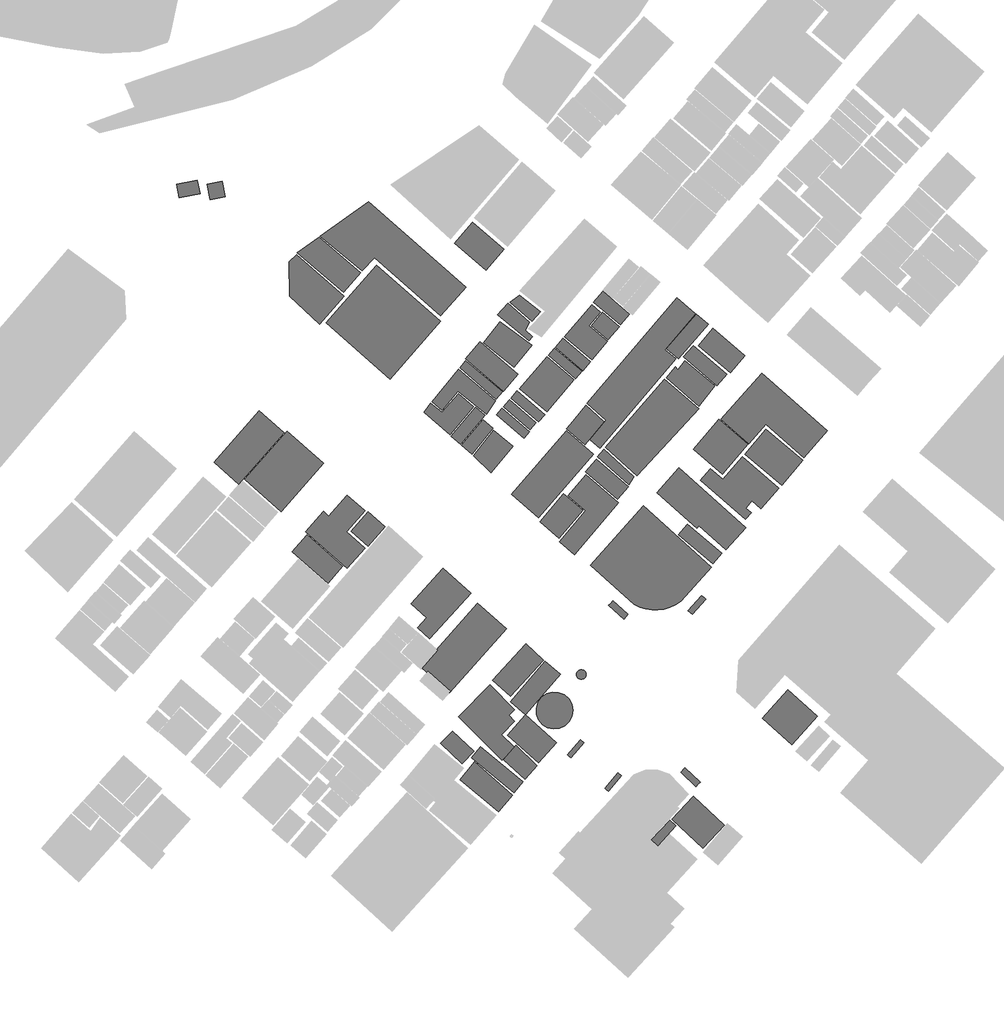
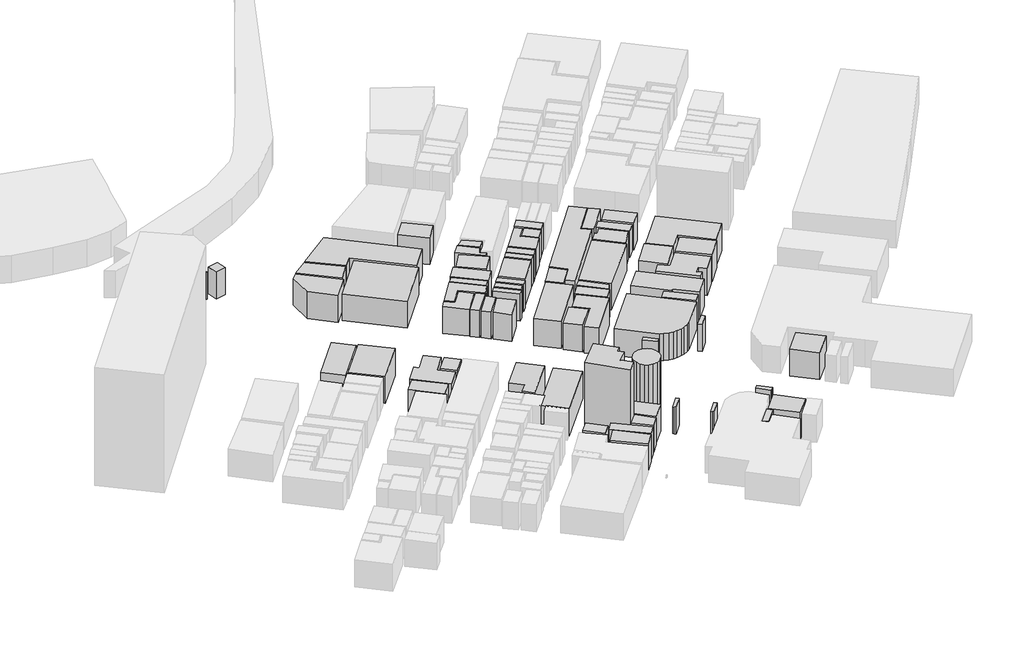
# One storey, part 2 of 3: 70 proxies.
"""IFC4 building model written with IfcOpenShell, lengths in millimetres."""

from ifc_helpers import new_model, si_unit, origin, origin_with_axes, place, context, project, spatial, polyline, outline, extrude, element, save

model = new_model("IFC4")

# Units and contexts
model_context = context("Model", 3, world=origin())
ifc_project = project(units=[si_unit("LENGTHUNIT", "METRE", prefix="MILLI")], contexts=[model_context])

# Site, building, storey
site = spatial("IfcSite", under=ifc_project)
building = spatial("IfcBuilding", under=site)
storey = spatial("IfcBuildingStorey", under=building, Name="レベル 0", Elevation=0.0)

# Proxies
placement = place(None, origin())
element("IfcBuildingElementProxy", 1, Name="Mass", at=placement, inside=storey, context=model_context, shape_type="SweptSolid", body=[
    extrude(outline(polyline([(170698.7323915, 46624.0327425), (171096.1893538, 44511.3291361), (170789.0635192, 42387.5060369), (169804.4542245, 40486.0727911), (168268.8250515, 38984.9412821), (166326.7058014, 38073.1428832), (164194.8911837, 37828.5140449), (162099.2090151, 38284.4132439), (160265.4871197, 39385.2430179), (158883.4208628, 41030.9279318), (158097.5400505, 43054.6755966), (158016.2420351, 45234.096159), (158657.593041, 47313.4412879), (159931.2619458, 49070.3211289), (161719.8182773, 50315.7043068), (163815.500446, 50905.0374178), (165983.4475152, 50782.7229987), (167997.8316659, 49959.8805414), (169623.7919691, 48514.3464955), (170698.7323915, 46624.0327425)])), origin_with_axes(), (0.0, 0.0, 1.0), 35000.0),
])
element("IfcBuildingElementProxy", 2, Name="Mass", at=placement, inside=storey, context=model_context, shape_type="SweptSolid", body=[
    extrude(outline(polyline([(130374.9168956, 42153.9966913), (141485.6456275, 53473.6402233), (150256.798147, 44678.1215256), (148287.5795602, 42676.6128464), (150310.9968231, 40486.0727911), (145677.0099623, 35793.6468872), (150175.5001316, 31245.7743872), (145848.6391053, 26586.7069609), (130374.9168956, 42153.9966913)])), origin_with_axes(), (0.0, 0.0, 1.0), 45000.0),
])
element("IfcBuildingElementProxy", 3, Name="Mass", at=placement, inside=storey, context=model_context, shape_type="SweptSolid", body=[
    extrude(outline(polyline([(208574.5743203, 165836.1135976), (210995.448548, 168927.3325589), (221636.4554144, 160031.7384269), (215927.5281312, 152781.8292102), (204419.3424371, 162933.9260122), (207608.0312501, 166803.5094596), (208574.5743203, 165836.1135976)])), origin_with_axes(), (0.0, 0.0, 1.0), 15000.0),
])
element("IfcBuildingElementProxy", 4, Name="Mass", at=placement, inside=storey, context=model_context, shape_type="SweptSolid", body=[
    extrude(outline(polyline([(177934.2557355, 188964.6583397), (180978.4147472, 186362.6970567), (176868.3484279, 181547.9567328), (183462.5207633, 175921.4934444), (177780.6928194, 169283.1563236), (168151.3945845, 177511.5808958), (177934.2557355, 188964.6583397)])), origin_with_axes(), (0.0, 0.0, 1.0), 15000.0),
])
element("IfcBuildingElementProxy", 5, Name="Mass", at=placement, inside=storey, context=model_context, shape_type="SweptSolid", body=[
    extrude(outline(polyline([(164809.1428529, 173875.5067947), (167519.0766882, 177044.562204), (177310.970954, 168671.5842278), (174601.0371162, 165502.5288177), (164809.1428529, 173875.5067947)])), origin_with_axes(), (0.0, 0.0, 1.0), 15000.0),
])
element("IfcBuildingElementProxy", 6, Name="Mass", at=placement, inside=storey, context=model_context, shape_type="SweptSolid", body=[
    extrude(outline(polyline([(146282.2285192, 152626.1563127), (148432.1093639, 155139.161655), (157980.1095835, 146988.5735315), (155830.2287387, 144475.5681892), (146282.2285192, 152626.1563127)])), origin_with_axes(), (0.0, 0.0, 1.0), 15000.0),
])
element("IfcBuildingElementProxy", 7, Name="Mass", at=placement, inside=storey, context=model_context, shape_type="SweptSolid", body=[
    extrude(outline(polyline([(247760.2176028, 51805.7163239), (258292.8271145, 42287.4306033), (249151.3169721, 32168.6922789), (238618.7074578, 41686.9779995), (247760.2176028, 51805.7163239)])), origin_with_axes(), (0.0, 0.0, 1.0), 15000.0),
])
element("IfcBuildingElementProxy", 8, Name="Mass", at=placement, inside=storey, context=model_context, shape_type="SweptSolid", body=[
    extrude(outline(polyline([(145125.990084, 182937.8933163), (156489.6459718, 174520.4373689), (150148.4007948, 166681.1950405), (139254.4667699, 175421.116275), (145125.990084, 182937.8933163)])), origin_with_axes(), (0.0, 0.0, 1.0), 15000.0),
])
element("IfcBuildingElementProxy", 9, Name="Mass", at=placement, inside=storey, context=model_context, shape_type="SweptSolid", body=[
    extrude(outline(polyline([(139028.6389507, 148000.447364), (142551.5529376, 144864.7504331), (135026.9699836, 135657.8105068), (131350.4930781, 138860.2243936), (139028.6389507, 148000.447364)])), origin_with_axes(), (0.0, 0.0, 1.0), 15000.0),
])
element("IfcBuildingElementProxy", 10, Name="Mass", at=placement, inside=storey, context=model_context, shape_type="SweptSolid", body=[
    extrude(outline(polyline([(215792.0314397, 174387.0034569), (221031.2368575, 180524.9634075), (232394.8927479, 170817.6463118), (227155.6873275, 164679.6863612), (215792.0314397, 174387.0034569)])), origin_with_axes(), (0.0, 0.0, 1.0), 15000.0),
])
element("IfcBuildingElementProxy", 11, Name="Mass", at=placement, inside=storey, context=model_context, shape_type="SweptSolid", body=[
    extrude(outline(polyline([(203868.3225562, 173008.1863662), (207725.4617171, 169716.8165378), (180707.4213617, 137803.8725908), (177220.6398263, 140939.5695225), (182839.2359819, 147878.1329448), (176109.5669524, 153916.0174618), (208177.117358, 191455.4246972), (214798.3890328, 185795.6029305), (203868.3225562, 173008.1863662)])), origin_with_axes(), (0.0, 0.0, 1.0), 15000.0),
])
element("IfcBuildingElementProxy", 12, Name="Mass", at=placement, inside=storey, context=model_context, shape_type="SweptSolid", body=[
    extrude(outline(polyline([(138025.9634289, 175721.3425765), (151422.0696971, 164268.2651325), (146246.0960676, 158219.2611227), (132849.9898021, 169672.3385674), (138025.9634289, 175721.3425765)])), origin_with_axes(), (0.0, 0.0, 1.0), 15000.0),
])
element("IfcBuildingElementProxy", 13, Name="Mass", at=placement, inside=storey, context=model_context, shape_type="SweptSolid", body=[
    extrude(outline(polyline([(162334.0699465, 170951.0802238), (164502.0170183, 173486.3245509), (174230.6794932, 165180.0635306), (172053.6993091, 162633.6997107), (162334.0699465, 170951.0802238)])), origin_with_axes(), (0.0, 0.0, 1.0), 15000.0),
])
element("IfcBuildingElementProxy", 14, Name="Mass", at=placement, inside=storey, context=model_context, shape_type="SweptSolid", body=[
    extrude(outline(polyline([(187355.7923757, 118344.7604281), (171556.8781069, 99930.8805755), (166218.3084467, 104512.1115531), (175630.8119747, 115475.9313204), (169334.732359, 120880.0047552), (175721.1431024, 128318.9453478), (187355.7923757, 118344.7604281)])), origin_with_axes(), (0.0, 0.0, 1.0), 15000.0),
])
element("IfcBuildingElementProxy", 15, Name="Mass", at=placement, inside=storey, context=model_context, shape_type="SweptSolid", body=[
    extrude(outline(polyline([(168792.745593, 144742.4360131), (170156.7456229, 146410.3599133), (175648.8781992, 153137.6529749), (182152.7194095, 147299.9193266), (175323.6861401, 139104.8532327), (168792.745593, 144742.4360131)])), origin_with_axes(), (0.0, 0.0, 1.0), 15000.0),
])
element("IfcBuildingElementProxy", 16, Name="Mass", at=placement, inside=storey, context=model_context, shape_type="SweptSolid", body=[
    extrude(outline(polyline([(144186.5463531, 185328.5842386), (147953.3543863, 189565.1109435), (155676.6658227, 182782.2204187), (154159.1028717, 179813.3158774), (156715.4737935, 177600.5368366), (155333.4075365, 176043.8078635), (144186.5463531, 185328.5842386)])), origin_with_axes(), (0.0, 0.0, 1.0), 15000.0),
])
element("IfcBuildingElementProxy", 17, Name="Mass", at=placement, inside=storey, context=model_context, shape_type="SweptSolid", body=[
    extrude(outline(polyline([(148956.0299055, 155661.77781), (151160.1094263, 158241.5001083), (161060.4010443, 149779.5661905), (158856.3215234, 147199.8438922), (148956.0299055, 155661.77781)])), origin_with_axes(), (0.0, 0.0, 1.0), 15000.0),
])
element("IfcBuildingElementProxy", 18, Name="Mass", at=placement, inside=storey, context=model_context, shape_type="SweptSolid", body=[
    extrude(outline(polyline([(182649.5406117, 138148.5768635), (203660.5609616, 162455.7878276), (216017.8592589, 151903.3892898), (193940.9315989, 128085.4360023), (182649.5406117, 138148.5768635)])), origin_with_axes(), (0.0, 0.0, 1.0), 15000.0),
])
element("IfcBuildingElementProxy", 19, Name="Mass", at=placement, inside=storey, context=model_context, shape_type="SweptSolid", body=[
    extrude(outline(polyline([(143852.3211792, 149790.6856833), (145812.5066538, 152081.3011721), (155622.4671441, 143697.2037031), (153662.2816695, 141395.4687215), (143852.3211792, 149790.6856833)])), origin_with_axes(), (0.0, 0.0, 1.0), 15000.0),
])
element("IfcBuildingElementProxy", 20, Name="Mass", at=placement, inside=storey, context=model_context, shape_type="SweptSolid", body=[
    extrude(outline(polyline([(130230.3870919, 157296.3432318), (135695.4203289, 152537.2003711), (127195.2611949, 142629.7324075), (117945.3536977, 150635.7671254), (120375.2610377, 153838.1810131), (124494.3604693, 150591.289155), (130230.3870919, 157296.3432318)])), origin_with_axes(), (0.0, 0.0, 1.0), 15000.0),
])
element("IfcBuildingElementProxy", 21, Name="Mass", at=placement, inside=storey, context=model_context, shape_type="SweptSolid", body=[
    extrude(outline(polyline([(120881.1153548, 154405.2751393), (130338.7844466, 166025.1449735), (143545.1953446, 154672.1429632), (140257.1422891, 150001.956044), (130149.0890765, 158152.5441667), (124367.8968926, 151447.4900899), (120881.1153548, 154405.2751393)])), origin_with_axes(), (0.0, 0.0, 1.0), 15000.0),
])
element("IfcBuildingElementProxy", 22, Name="Mass", at=placement, inside=storey, context=model_context, shape_type="SweptSolid", body=[
    extrude(outline(polyline([(177654.2292402, 181525.7177472), (181682.9975441, 186251.5021295), (187644.8519858, 181158.7744897), (183607.0505671, 176444.1096002), (177654.2292402, 181525.7177472)])), origin_with_axes(), (0.0, 0.0, 1.0), 15000.0),
])
element("IfcBuildingElementProxy", 23, Name="Mass", at=placement, inside=storey, context=model_context, shape_type="SweptSolid", body=[
    extrude(outline(polyline([(142849.64566, 144219.8198581), (149778.0431693, 138471.0421506), (141955.3674929, 129052.8318643), (135659.2878798, 135157.4333365), (142849.64566, 144219.8198581)])), origin_with_axes(), (0.0, 0.0, 1.0), 15000.0),
])
element("IfcBuildingElementProxy", 24, Name="Mass", at=placement, inside=storey, context=model_context, shape_type="SweptSolid", body=[
    extrude(outline(polyline([(231563.8463692, 134768.2510935), (244463.1314351, 123582.0414727), (238121.8862556, 116276.5347921), (234933.1974401, 119034.1689735), (232765.2503708, 116532.283124), (234617.0384932, 114919.9566878), (232530.3894394, 112518.1462718), (216550.8129127, 126384.1536245), (220164.0580298, 130542.8438806), (224581.2501837, 126717.7384044), (231563.8463692, 134768.2510935)])), origin_with_axes(), (0.0, 0.0, 1.0), 15000.0),
])
element("IfcBuildingElementProxy", 25, Name="Mass", at=placement, inside=storey, context=model_context, shape_type="SweptSolid", body=[
    extrude(outline(polyline([(192902.1236281, 82150.8118051), (177265.8053902, 96139.1335769), (196163.0773468, 117277.2891325), (220516.3494282, 95494.2030027), (209559.183615, 83240.5220863), (207707.3954926, 82039.6168787), (205693.0113393, 81116.6989878), (203579.2629461, 80505.1268912), (201393.2496524, 80193.7810962), (199180.1370193, 80216.0200818), (197003.1568352, 80549.6048616), (194889.4084421, 81205.6549286), (192902.1236281, 82150.8118051)])), origin_with_axes(), (0.0, 0.0, 1.0), 15000.0),
])
element("IfcBuildingElementProxy", 26, Name="Mass", at=placement, inside=storey, context=model_context, shape_type="SweptSolid", body=[
    extrude(outline(polyline([(200959.6602385, 121969.7150364), (208881.7001549, 130854.1896757), (232729.1179192, 109571.4807161), (225656.1906061, 101654.4019389), (216053.9917105, 110216.4112902), (215204.8791073, 109260.134921), (200959.6602385, 121969.7150364)])), origin_with_axes(), (0.0, 0.0, 1.0), 15000.0),
])
element("IfcBuildingElementProxy", 27, Name="Mass", at=placement, inside=storey, context=model_context, shape_type="SweptSolid", body=[
    extrude(outline(polyline([(175567.5801838, 129464.2530922), (179424.7193472, 133923.1696506), (190842.5739136, 124060.1796573), (186994.4678651, 119601.2630989), (175567.5801838, 129464.2530922)])), origin_with_axes(), (0.0, 0.0, 1.0), 15000.0),
])
element("IfcBuildingElementProxy", 28, Name="Mass", at=placement, inside=storey, context=model_context, shape_type="SweptSolid", body=[
    extrude(outline(polyline([(161204.930848, 61913.3351563), (166579.6329599, 57298.7457003), (154249.4340019, 42943.4806703), (148874.73189, 47558.0701262), (161204.930848, 61913.3351563)])), origin_with_axes(), (0.0, 0.0, 1.0), 15000.0),
])
element("IfcBuildingElementProxy", 29, Name="Mass", at=placement, inside=storey, context=model_context, shape_type="SweptSolid", body=[
    extrude(outline(polyline([(130916.9036642, 19659.2630314), (135975.4468267, 26086.3297907), (149488.9835592, 14199.5921325), (144493.6721877, 8317.380513), (130916.9036642, 19659.2630314)])), origin_with_axes(), (0.0, 0.0, 1.0), 15000.0),
])
element("IfcBuildingElementProxy", 30, Name="Mass", at=placement, inside=storey, context=model_context, shape_type="SweptSolid", body=[
    extrude(outline(polyline([(116861.3801631, 59822.8705346), (137149.751489, 82651.1889753), (147465.5662963, 73488.7270194), (127177.1949678, 50660.4085795), (116861.3801631, 59822.8705346)])), origin_with_axes(), (0.0, 0.0, 1.0), 15000.0),
])
element("IfcBuildingElementProxy", 31, Name="Mass", at=placement, inside=storey, context=model_context, shape_type="SweptSolid", body=[
    extrude(outline(polyline([(123961.4068155, 32624.5914779), (128098.5724742, 37050.149558), (135749.6190075, 29889.1962821), (131621.4864611, 25463.6382021), (123961.4068155, 32624.5914779)])), origin_with_axes(), (0.0, 0.0, 1.0), 15000.0),
])
element("IfcBuildingElementProxy", 32, Name="Mass", at=placement, inside=storey, context=model_context, shape_type="SweptSolid", body=[
    extrude(outline(polyline([(69220.7433079, 143930.7130486), (82255.5250653, 132444.2771263), (67134.094254, 115275.7804524), (54099.3124992, 126762.2163747), (69220.7433079, 143930.7130486)])), origin_with_axes(), (0.0, 0.0, 1.0), 15000.0),
])
element("IfcBuildingElementProxy", 33, Name="Mass", at=placement, inside=storey, context=model_context, shape_type="SweptSolid", body=[
    extrude(outline(polyline([(40612.8751034, 231952.6169812), (45987.5772127, 232975.6103056), (47044.451408, 227426.983466), (41678.7824109, 226403.9901416), (40612.8751034, 231952.6169812)])), origin_with_axes(), (0.0, 0.0, 1.0), 15000.0),
])
element("IfcBuildingElementProxy", 34, Name="Mass", at=placement, inside=storey, context=model_context, shape_type="SweptSolid", body=[
    extrude(outline(polyline([(29809.2722061, 231885.9000252), (37198.3584687, 233353.6730567), (38155.868424, 228538.9327328), (30766.7821615, 227071.1597013), (29809.2722061, 231885.9000252)])), origin_with_axes(), (0.0, 0.0, 1.0), 15000.0),
])
element("IfcBuildingElementProxy", 35, Name="Mass", at=placement, inside=storey, context=model_context, shape_type="SweptSolid", body=[
    extrude(outline(polyline([(213976.3757689, 13832.6488751), (225105.1707253, 3547.1181603), (217481.2235313, -4703.5453967), (206352.4285723, 5581.985318), (213976.3757689, 13832.6488751)])), origin_with_axes(), (0.0, 0.0, 1.0), 15000.0),
])
element("IfcBuildingElementProxy", 36, Name="Mass", at=placement, inside=storey, context=model_context, shape_type="SweptSolid", body=[
    extrude(outline(polyline([(199125.9383406, -1756.879841), (205584.6139871, 5292.8785085), (207788.693508, 3269.1308436), (201339.0509737, -3780.6275059), (199125.9383406, -1756.879841)])), origin_with_axes(), (0.0, 0.0, 1.0), 15000.0),
])
element("IfcBuildingElementProxy", 37, Name="Mass", at=placement, inside=storey, context=model_context, shape_type="SweptSolid", body=[
    extrude(outline(polyline([(90367.2603492, 108081.468699), (96970.4657995, 102265.9740355), (90647.286847, 95082.781774), (75823.9487581, 108137.0661622), (82156.1608228, 115320.2584236), (84053.114509, 113652.3345234), (90593.088171, 121080.1556232), (96907.2340111, 115509.2897988), (90367.2603492, 108081.468699)])), origin_with_axes(), (0.0, 0.0, 1.0), 15000.0),
])
element("IfcBuildingElementProxy", 38, Name="Mass", at=placement, inside=storey, context=model_context, shape_type="SweptSolid", body=[
    extrude(outline(polyline([(216442.4155605, 18847.5400669), (215647.5016334, 18035.8171024), (214861.6208211, 17224.0941378), (209514.0180486, 22416.897212), (211094.8127879, 24040.343141), (216442.4155605, 18847.5400669)])), origin_with_axes(), (0.0, 0.0, 1.0), 15000.0),
])
element("IfcBuildingElementProxy", 39, Name="Mass", at=placement, inside=storey, context=model_context, shape_type="SweptSolid", body=[
    extrude(outline(polyline([(174944.2954023, 58722.0407614), (175404.9841555, 58343.9780104), (175712.1099901, 57821.3618554), (175811.47423, 57220.9092516), (175712.1099901, 56631.5761406), (175414.0172678, 56097.8404928), (174962.3616268, 55708.6582489), (174393.2755215, 55497.3878882), (173842.2556432, 55475.1489034), (173318.3350991, 55630.8218001), (172857.6463485, 55942.1675952), (172523.4211746, 56386.9473015), (172342.7589192, 56909.5634573), (172333.725807, 57454.4185979), (172496.3218352, 57988.1542457), (172812.4807847, 58432.9339519), (173255.1033108, 58766.5187318), (173779.0238523, 58944.4306142), (174375.209297, 58933.3111222), (174944.2954023, 58722.0407614)])), origin_with_axes(), (0.0, 0.0, 1.0), 15000.0),
])
element("IfcBuildingElementProxy", 40, Name="Mass", at=placement, inside=storey, context=model_context, shape_type="SweptSolid", body=[
    extrude(outline(polyline([(213642.150595, 78648.1716159), (212151.6869832, 79971.3912426), (216939.2367627, 85353.2256927), (217725.117575, 84663.8171474), (218429.7003744, 84041.125558), (213642.150595, 78648.1716159)])), origin_with_axes(), (0.0, 0.0, 1.0), 15000.0),
])
element("IfcBuildingElementProxy", 41, Name="Mass", at=placement, inside=storey, context=model_context, shape_type="SweptSolid", body=[
    extrude(outline(polyline([(223126.9190236, 148089.4033055), (233424.6676038, 139227.1676519), (224310.2568007, 128630.2911429), (214003.4751057, 137492.5267965), (223126.9190236, 148089.4033055)])), origin_with_axes(), (0.0, 0.0, 1.0), 15000.0),
])
element("IfcBuildingElementProxy", 42, Name="Mass", at=placement, inside=storey, context=model_context, shape_type="SweptSolid", body=[
    extrude(outline(polyline([(146264.1622947, 26875.8137704), (150753.6193518, 32024.1388742), (158260.1360788, 24640.7957448), (154077.8048588, 19859.4138993), (146264.1622947, 26875.8137704)])), origin_with_axes(), (0.0, 0.0, 1.0), 15000.0),
])
element("IfcBuildingElementProxy", 43, Name="Mass", at=placement, inside=storey, context=model_context, shape_type="SweptSolid", body=[
    extrude(outline(polyline([(187066.7327657, 22172.2683729), (188340.4016705, 21082.5580917), (183688.3485825, 15634.0066864), (183056.0306888, 16178.861827), (182414.6796803, 16723.7169676), (187066.7327657, 22172.2683729)])), origin_with_axes(), (0.0, 0.0, 1.0), 15000.0),
])
element("IfcBuildingElementProxy", 44, Name="Mass", at=placement, inside=storey, context=model_context, shape_type="SweptSolid", body=[
    extrude(outline(polyline([(185296.2426587, 83418.4339686), (190761.2758982, 78603.6936455), (189288.8785136, 76935.7697453), (183778.6797102, 81828.346518), (184573.5936373, 82662.3084681), (185296.2426587, 83418.4339686)])), origin_with_axes(), (0.0, 0.0, 1.0), 15000.0),
])
element("IfcBuildingElementProxy", 45, Name="Mass", at=placement, inside=storey, context=model_context, shape_type="SweptSolid", body=[
    extrude(outline(polyline([(173760.9576278, 33981.1695831), (175034.62653, 32902.5787946), (170382.5734446, 27454.0273886), (169623.7919691, 28098.9579636), (169117.9376521, 28532.618177), (173760.9576278, 33981.1695831)])), origin_with_axes(), (0.0, 0.0, 1.0), 15000.0),
])
element("IfcBuildingElementProxy", 46, Name="Mass", at=placement, inside=storey, context=model_context, shape_type="SweptSolid", body=[
    extrude(outline(polyline([(158865.3546357, 25697.1475476), (147727.5265671, 35537.8985561), (154141.0366472, 42798.9272655), (165278.8647184, 32947.056765), (158865.3546357, 25697.1475476)])), origin_with_axes(), (0.0, 0.0, 1.0), 15000.0),
])
element("IfcBuildingElementProxy", 47, Name="Mass", at=placement, inside=storey, context=model_context, shape_type="SweptSolid", body=[
    extrude(outline(polyline([(211844.5611486, 110716.7884605), (224165.7269944, 100497.9747017), (221004.1375182, 96683.9887175), (208692.0047847, 106913.921969), (211844.5611486, 110716.7884605)])), origin_with_axes(), (0.0, 0.0, 1.0), 15000.0),
])
element("IfcBuildingElementProxy", 48, Name="Mass", at=placement, inside=storey, context=model_context, shape_type="SweptSolid", body=[
    extrude(outline(polyline([(118966.095444, 77458.3859011), (113392.6648523, 82495.5160777), (124801.4863065, 95105.0207596), (134665.6454729, 86176.06815), (119932.6385116, 69908.2503814), (115650.9430492, 73788.9533216), (118966.095444, 77458.3859011)])), origin_with_axes(), (0.0, 0.0, 1.0), 15000.0),
])
element("IfcBuildingElementProxy", 49, Name="Mass", at=placement, inside=storey, context=model_context, shape_type="SweptSolid", body=[
    extrude(outline(polyline([(142470.2549222, 55230.5200643), (154339.7651296, 68106.8925701), (160644.8778549, 62302.5173993), (148775.3676501, 49415.0254008), (142470.2549222, 55230.5200643)])), origin_with_axes(), (0.0, 0.0, 1.0), 15000.0),
])
element("IfcBuildingElementProxy", 50, Name="Mass", at=placement, inside=storey, context=model_context, shape_type="SweptSolid", body=[
    extrude(outline(polyline([(138071.1289928, 31434.8057624), (153264.8247072, 18925.3765148), (150040.0034401, 15011.315097), (134846.3077282, 27520.7443446), (138071.1289928, 31434.8057624)])), origin_with_axes(), (0.0, 0.0, 1.0), 15000.0),
])
element("IfcBuildingElementProxy", 51, Name="Mass", at=placement, inside=storey, context=model_context, shape_type="SweptSolid", body=[
    extrude(outline(polyline([(239829.1445717, 144520.0461604), (252972.3236813, 133467.2704515), (245610.3367581, 124716.2297251), (232467.1576485, 135769.0054331), (239829.1445717, 144520.0461604)])), origin_with_axes(), (0.0, 0.0, 1.0), 15000.0),
])
element("IfcBuildingElementProxy", 52, Name="Mass", at=placement, inside=storey, context=model_context, shape_type="SweptSolid", body=[
    extrude(outline(polyline([(98189.9360256, 225692.3426106), (132922.2547027, 195247.1716951), (123916.2412517, 184972.7604732), (100312.717531, 205766.2117561), (95895.5253771, 201051.5468666), (80972.8230482, 213349.7057534), (98189.9360256, 225692.3426106)])), origin_with_axes(), (0.0, 0.0, 1.0), 15000.0),
])
element("IfcBuildingElementProxy", 53, Name="Mass", at=placement, inside=storey, context=model_context, shape_type="SweptSolid", body=[
    extrude(outline(polyline([(204491.6073377, 173230.5762197), (215096.4817551, 185639.9300337), (219305.9123144, 182037.2144102), (208692.0047847, 169627.8605962), (204491.6073377, 173230.5762197)])), origin_with_axes(), (0.0, 0.0, 1.0), 15000.0),
])
element("IfcBuildingElementProxy", 54, Name="Mass", at=placement, inside=storey, context=model_context, shape_type="SweptSolid", body=[
    extrude(outline(polyline([(132877.0891388, 168949.5715437), (146011.2351362, 157930.1543132), (143680.6920361, 155216.9981038), (130745.2745212, 166481.0441726), (132877.0891388, 168949.5715437)])), origin_with_axes(), (0.0, 0.0, 1.0), 15000.0),
])
element("IfcBuildingElementProxy", 55, Name="Mass", at=placement, inside=storey, context=model_context, shape_type="SweptSolid", body=[
    extrude(outline(polyline([(127556.5857056, 142184.9527004), (136354.8375645, 152470.4834152), (139742.2548598, 149579.4153226), (130953.0361158, 139293.8846079), (127556.5857056, 142184.9527004)])), origin_with_axes(), (0.0, 0.0, 1.0), 15000.0),
])
element("IfcBuildingElementProxy", 56, Name="Mass", at=placement, inside=storey, context=model_context, shape_type="SweptSolid", body=[
    extrude(outline(polyline([(159262.811598, 111717.5428001), (167799.103186, 121602.771779), (174655.2357922, 115676.0821883), (166118.9442067, 105790.8532102), (159262.811598, 111717.5428001)])), origin_with_axes(), (0.0, 0.0, 1.0), 15000.0),
])
element("IfcBuildingElementProxy", 57, Name="Mass", at=placement, inside=storey, context=model_context, shape_type="SweptSolid", body=[
    extrude(outline(polyline([(92011.2868769, 108203.7831182), (98099.6048979, 115108.9880629), (104088.558679, 109827.2290472), (98000.240658, 102922.0241024), (92011.2868769, 108203.7831182)])), origin_with_axes(), (0.0, 0.0, 1.0), 15000.0),
])
element("IfcBuildingElementProxy", 58, Name="Mass", at=placement, inside=storey, context=model_context, shape_type="SweptSolid", body=[
    extrude(outline(polyline([(43115.0473466, 132766.7424142), (59284.3192409, 151125.0248028), (68046.4386456, 143408.0968936), (51877.1667513, 125049.8145049), (43115.0473466, 132766.7424142)])), origin_with_axes(), (0.0, 0.0, 1.0), 15000.0),
])
element("IfcBuildingElementProxy", 59, Name="Mass", at=placement, inside=storey, context=model_context, shape_type="SweptSolid", body=[
    extrude(outline(polyline([(80602.4654227, 213005.0014807), (95326.4392717, 200428.8552772), (89301.3530417, 193367.977435), (72788.8228612, 207467.4941339), (80602.4654227, 213005.0014807)])), origin_with_axes(), (0.0, 0.0, 1.0), 15000.0),
])
element("IfcBuildingElementProxy", 60, Name="Mass", at=placement, inside=storey, context=model_context, shape_type="SweptSolid", body=[
    extrude(outline(polyline([(128902.519511, 210814.4614255), (135343.1289304, 218320.118974), (146535.1556777, 208723.9968047), (140094.5462583, 201218.3392562), (128902.519511, 210814.4614255)])), origin_with_axes(), (0.0, 0.0, 1.0), 15000.0),
])
element("IfcBuildingElementProxy", 61, Name="Mass", at=placement, inside=storey, context=model_context, shape_type="SweptSolid", body=[
    extrude(outline(polyline([(210552.8260193, 170361.7471128), (213958.3095418, 174353.6449785), (225900.0846498, 164157.0702054), (222485.5680151, 160165.1723388), (210552.8260193, 170361.7471128)])), origin_with_axes(), (0.0, 0.0, 1.0), 15000.0),
])
element("IfcBuildingElementProxy", 62, Name="Mass", at=placement, inside=storey, context=model_context, shape_type="SweptSolid", body=[
    extrude(outline(polyline([(148712.1358592, 189787.500797), (152072.4538178, 192344.9841097), (159461.5400804, 186485.0114758), (156489.6459718, 183149.1636762), (148712.1358592, 189787.500797)])), origin_with_axes(), (0.0, 0.0, 1.0), 15000.0),
])
element("IfcBuildingElementProxy", 63, Name="Mass", at=placement, inside=storey, context=model_context, shape_type="SweptSolid", body=[
    extrude(outline(polyline([(149172.8246124, 121358.1429399), (168702.4144653, 143975.1910198), (178340.7458125, 135668.9299996), (158811.1559596, 113051.8819196), (149172.8246124, 121358.1429399)])), origin_with_axes(), (0.0, 0.0, 1.0), 15000.0),
])
element("IfcBuildingElementProxy", 64, Name="Mass", at=placement, inside=storey, context=model_context, shape_type="SweptSolid", body=[
    extrude(outline(polyline([(101035.366555, 203019.6970675), (123834.9432363, 183026.849257), (105831.9494467, 162489.146306), (83032.3727653, 182470.8746236), (101035.366555, 203019.6970675)])), origin_with_axes(), (0.0, 0.0, 1.0), 15000.0),
])
element("IfcBuildingElementProxy", 65, Name="Mass", at=placement, inside=storey, context=model_context, shape_type="SweptSolid", body=[
    extrude(outline(polyline([(72544.9288149, 206811.4440662), (89482.015297, 192055.877301), (80801.1939052, 182081.6923806), (70133.0876994, 191944.6823739), (69889.1936557, 204365.1556806), (72544.9288149, 206811.4440662)])), origin_with_axes(), (0.0, 0.0, 1.0), 15000.0),
])
element("IfcBuildingElementProxy", 66, Name="Mass", at=placement, inside=storey, context=model_context, shape_type="SweptSolid", body=[
    extrude(outline(polyline([(178476.2425041, 189898.6957242), (181728.1631079, 193701.5622148), (191221.9646488, 185595.4520625), (187970.0440449, 181781.4660791), (178476.2425041, 189898.6957242)])), origin_with_axes(), (0.0, 0.0, 1.0), 15000.0),
])
element("IfcBuildingElementProxy", 67, Name="Mass", at=placement, inside=storey, context=model_context, shape_type="SweptSolid", body=[
    extrude(outline(polyline([(152072.4538178, 159086.5815504), (161774.016956, 170428.4640687), (171439.4476399, 162166.6810189), (161746.9176166, 150824.7985005), (152072.4538178, 159086.5815504)])), origin_with_axes(), (0.0, 0.0, 1.0), 15000.0),
])
element("IfcBuildingElementProxy", 68, Name="Mass", at=placement, inside=storey, context=model_context, shape_type="SweptSolid", body=[
    extrude(outline(polyline([(182179.8187463, 137503.6462893), (192911.156743, 127729.6122368), (191068.4017328, 124738.4687099), (179758.9445185, 134790.4900791), (182179.8187463, 137503.6462893)])), origin_with_axes(), (0.0, 0.0, 1.0), 15000.0),
])
element("IfcBuildingElementProxy", 69, Name="Mass", at=placement, inside=storey, context=model_context, shape_type="SweptSolid", body=[
    extrude(outline(polyline([(238356.747187, 164635.20839), (261779.6086524, 144053.0274686), (253378.8137584, 134490.2637768), (239883.3432503, 146354.7624501), (233840.1907932, 139471.7964902), (223912.7998359, 148200.5982319), (238356.747187, 164635.20839)])), origin_with_axes(), (0.0, 0.0, 1.0), 15000.0),
])
element("IfcBuildingElementProxy", 70, Name="Mass", at=placement, inside=storey, context=model_context, shape_type="SweptSolid", body=[
    extrude(outline(polyline([(76257.538172, 106925.0414618), (88994.2272071, 95705.4733634), (83782.121126, 89801.0227583), (71054.4652058, 101009.4713639), (76257.538172, 106925.0414618)])), origin_with_axes(), (0.0, 0.0, 1.0), 15000.0),
])

save(model, "model.ifc")

# Revit data of these elements
# Elements 1, 2, 3, 4, 5, 6, 7, 8, 9, 10, 11, 12, 13, 14, 15, 16, 17, 18, 19, 20, 21, 22, 23, 24, 25, 26, 27, 28, 29, 30, 31, 32, 33, 34, 35, 36, 37, 38, 39, 40, 41, 42, 43, 44, 45, 46, 47, 48, 49, 50, 51, 52, 53, 54, 55, 56, 57, 58, 59, 60, 61, 62, 63, 64, 65, 66, 67, 68, 69, 70 (IfcBuildingElementProxy)
#   Phase Created = 新しい建設
#   Materials on its faces: "周辺建物"
# Materials
#   "周辺建物": class "一般", colour RGB 120 120 120, transparency 0, Cost = 0
